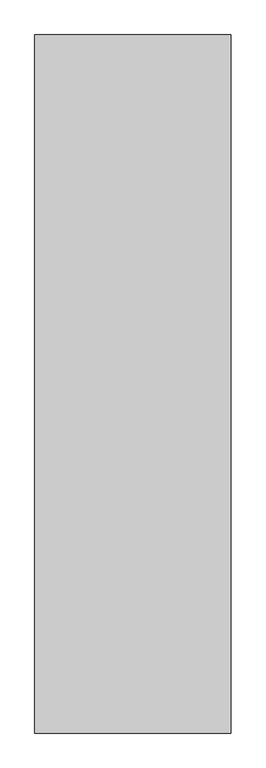
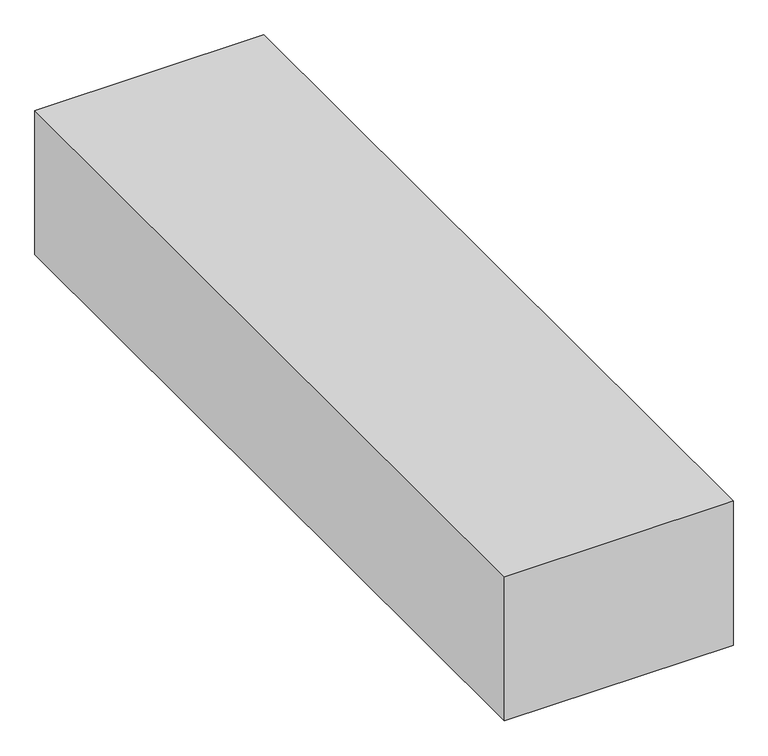
"""IFC4 building model written with IfcOpenShell, lengths in millimetres: proxy geometry, Space Planning Box_hec : Space Planning Box_hec."""

import ifcopenshell
import ifcopenshell.guid

model = None  # the IFC model being written
_history = None  # IfcOwnerHistory: only IFC2X3 demands one
_inside = {}  # id of a spatial element -> (the spatial element, [elements in it])
_under = {}  # id of a project, library or spatial element -> (it, [spatial elements below it])
_declared = {}  # id of a project -> (the project, [libraries it declares])
_typed = {}  # id of a type object -> (the type object, [elements of that type])
_made_of = {}  # id of a material, layer set ... -> (it, [elements and type objects made of it])


def new_model(schema):
    """Start an empty IFC model of exactly this schema.

    Asked for "IFC4X3", IfcOpenShell would pick the latest addendum, in which some entities
    have other attributes; the version numbers below select the first issue.
    IFC2X3 requires an IfcOwnerHistory on every rooted entity: one is made here for all.
    """
    global model, _history
    if schema == "IFC4X3":
        model = ifcopenshell.file(schema_version=(4, 3, 0, 0))
    else:
        model = ifcopenshell.file(schema=schema)
    _inside.clear()
    _under.clear()
    _declared.clear()
    _typed.clear()
    _made_of.clear()
    _history = None
    if model.schema == "IFC2X3":
        org = make("IfcOrganization", Name="unknown")
        user = make(
            "IfcPersonAndOrganization",
            ThePerson=make("IfcPerson", FamilyName="unknown"),
            TheOrganization=org,
        )
        app = make(
            "IfcApplication",
            ApplicationDeveloper=org,
            Version="unknown",
            ApplicationFullName="unknown",
            ApplicationIdentifier="unknown",
        )
        _history = make(
            "IfcOwnerHistory",
            OwningUser=user,
            OwningApplication=app,
            ChangeAction="ADDED",
            CreationDate=0,
        )
    return model


def make(cls, **values):
    """One entity of the class cls with the attributes given. An attribute that is None is left unset."""
    return model.create_entity(
        cls, **{name: value for name, value in values.items() if value is not None}
    )


def rooted(cls, **values):
    """An entity with a GlobalId (a new one), such as an element, a storey or a relation."""
    return make(cls, GlobalId=ifcopenshell.guid.new(), OwnerHistory=_history, **values)


def si_unit(unit_type, name, prefix=None):
    """IfcSIUnit, for example si_unit("LENGTHUNIT", "METRE", prefix="MILLI")."""
    return make("IfcSIUnit", UnitType=unit_type, Prefix=prefix, Name=name)


def assignment(units):
    """IfcUnitAssignment: the units of a project."""
    return None if units is None else make("IfcUnitAssignment", Units=units)


def point(xyz):
    """IfcCartesianPoint."""
    return None if xyz is None else make("IfcCartesianPoint", Coordinates=xyz)


def direction(xyz):
    """IfcDirection."""
    return None if xyz is None else make("IfcDirection", DirectionRatios=xyz)


def frame(location, z_axis=None, x_axis=None):
    """IfcAxis2Placement3D, a coordinate frame: its origin and axes. An axis left out is left unset."""
    return make(
        "IfcAxis2Placement3D",
        Location=point(location),
        Axis=direction(z_axis),
        RefDirection=direction(x_axis),
    )


def origin():
    """The frame at (0, 0, 0) with its axes left unset."""
    return frame((0.0, 0.0, 0.0))


def origin_with_axes():
    """The frame at (0, 0, 0) with the z axis (0, 0, 1) and the x axis (1, 0, 0) written out."""
    return frame((0.0, 0.0, 0.0), z_axis=(0.0, 0.0, 1.0), x_axis=(1.0, 0.0, 0.0))


def place(relative_to, where):
    """IfcLocalPlacement: puts the frame where relative to a parent placement (None: the world)."""
    return make(
        "IfcLocalPlacement", PlacementRelTo=relative_to, RelativePlacement=where
    )


def context(
    kind, dimensions, precision=None, world=None, true_north=None, identifier=None
):
    """IfcGeometricRepresentationContext, for example the 3D "Model" context."""
    return make(
        "IfcGeometricRepresentationContext",
        ContextIdentifier=identifier,
        ContextType=kind,
        CoordinateSpaceDimension=dimensions,
        Precision=precision,
        WorldCoordinateSystem=world,
        TrueNorth=true_north,
    )


def project(units=None, contexts=None):
    """IfcProject with its units and contexts."""
    return rooted(
        "IfcProject",
        Name="project",
        RepresentationContexts=contexts,
        UnitsInContext=assignment(units),
    )


def spatial(cls, under=None, at=None, **own):
    """A site, building, storey or space (cls), placed at a placement, below another one or the project."""
    s = rooted(cls, ObjectPlacement=at, **own)
    if under is not None:
        _under.setdefault(under.id(), (under, []))[1].append(s)
    return s


def polyline(points):
    """IfcPolyline through the points."""
    return make("IfcPolyline", Points=[point(p) for p in points])


def outline(outer, holes=None, kind="AREA"):
    """IfcArbitraryClosedProfileDef: a profile drawn as a closed curve; with holes, ...WithVoids."""
    if holes is None:
        return make("IfcArbitraryClosedProfileDef", ProfileType=kind, OuterCurve=outer)
    return make(
        "IfcArbitraryProfileDefWithVoids",
        ProfileType=kind,
        OuterCurve=outer,
        InnerCurves=holes,
    )


def extrude(swept, where, along, depth):
    """IfcExtrudedAreaSolid: the profile swept, set in the frame where, extruded along a direction by depth."""
    return make(
        "IfcExtrudedAreaSolid",
        SweptArea=swept,
        Position=where,
        ExtrudedDirection=direction(along),
        Depth=depth,
    )


def shape(context_of_items, identifier, shape_type, items):
    """IfcShapeRepresentation: the items that make up one representation, for example the "Body"."""
    return make(
        "IfcShapeRepresentation",
        ContextOfItems=context_of_items,
        RepresentationIdentifier=identifier,
        RepresentationType=shape_type,
        Items=items,
    )


def source(mapping_origin, context_of_items, identifier, shape_type, items):
    """IfcRepresentationMap: a shape defined once, which mapped items show again and again."""
    return make(
        "IfcRepresentationMap",
        MappingOrigin=mapping_origin,
        MappedRepresentation=shape(context_of_items, identifier, shape_type, items),
    )


def transform(
    local_origin,
    x_axis=None,
    y_axis=None,
    z_axis=None,
    scale=None,
    scale2=None,
    scale3=None,
    uniform=True,
):
    """IfcCartesianTransformationOperator3D, or its non-uniform kind. x_axis, y_axis, z_axis: its Axis1, 2, 3."""
    if uniform:
        return make(
            "IfcCartesianTransformationOperator3D",
            Axis1=direction(x_axis),
            Axis2=direction(y_axis),
            LocalOrigin=point(local_origin),
            Scale=scale,
            Axis3=direction(z_axis),
        )
    return make(
        "IfcCartesianTransformationOperator3DnonUniform",
        Axis1=direction(x_axis),
        Axis2=direction(y_axis),
        LocalOrigin=point(local_origin),
        Scale=scale,
        Axis3=direction(z_axis),
        Scale2=scale2,
        Scale3=scale3,
    )


def mapped(mapping_source, mapping_target):
    """IfcMappedItem: shows the shape of a source again, moved by a transform."""
    return make(
        "IfcMappedItem", MappingSource=mapping_source, MappingTarget=mapping_target
    )


def made_of(thing, what):
    """Note that an element or type object is made of a material, layer set ...; save() writes the relation."""
    if what is not None:
        _made_of.setdefault(what.id(), (what, []))[1].append(thing)
    return thing


def element(
    cls,
    number,
    at=None,
    inside=None,
    cuts=None,
    type_object=None,
    material=None,
    context=None,
    identifier="Body",
    shape_type=None,
    held_by="IfcProductDefinitionShape",
    body=None,
    shapes=None,
    **own,
):
    """One element of the class cls, such as IfcWall. Its Tag is "e" and its number.

    at: its placement. inside: the storey or other place that contains it. cuts: it is an
    opening in that element (IfcRelVoidsElement). A single representation is given by context,
    identifier, shape_type and body (its items); several are given by shapes. held_by: the class
    of the entity that holds the representations. save() writes the other relations.
    """
    e = rooted(cls, Tag="e%d" % number, ObjectPlacement=at, **own)
    if body is not None:
        shapes = [shape(context, identifier, shape_type, body)]
    if shapes is not None:
        e.Representation = make(held_by, Representations=shapes)
    if inside is not None:
        _inside.setdefault(inside.id(), (inside, []))[1].append(e)
    if cuts is not None:
        rooted(
            "IfcRelVoidsElement", RelatingBuildingElement=cuts, RelatedOpeningElement=e
        )
    if type_object is not None:
        _typed.setdefault(type_object.id(), (type_object, []))[1].append(e)
    return made_of(e, material)


def aggregate(whole, parts):
    """IfcRelAggregates: a whole, such as a stair, and the parts it consists of."""
    return rooted("IfcRelAggregates", RelatingObject=whole, RelatedObjects=parts)


def save(model, path):
    """Write the relations noted so far, then the file.

    IfcRelAggregates (storeys below a building ...), IfcRelContainedInSpatialStructure (elements
    in a storey), IfcRelDefinesByType, IfcRelAssociatesMaterial and IfcRelDeclares: one each for
    every whole, place, type object, material and project.
    """
    for whole, parts in _under.values():
        aggregate(whole, parts)
    for where, things in _inside.values():
        rooted(
            "IfcRelContainedInSpatialStructure",
            RelatedElements=things,
            RelatingStructure=where,
        )
    for kind, things in _typed.values():
        rooted("IfcRelDefinesByType", RelatedObjects=things, RelatingType=kind)
    for what, things in _made_of.values():
        rooted("IfcRelAssociatesMaterial", RelatedObjects=things, RelatingMaterial=what)
    for by, libraries in _declared.values():
        rooted("IfcRelDeclares", RelatingContext=by, RelatedDefinitions=libraries)
    model.write(path)


def generic_models_57c7875f(model_context):
    return source(origin(), model_context, "Body", "SweptSolid", [
        extrude(outline(polyline([(4500.0, 16000.0), (4500.0, -16000.0), (-4500.0, -16000.0), (-4500.0, 16000.0), (4500.0, 16000.0)])), origin_with_axes(), (0.0, 0.0, 1.0), 6000.0),
    ])


if __name__ == "__main__":
    model = new_model("IFC4")
    model_context = context("Model", 3, world=origin())
    ifc_project = project(units=[si_unit("LENGTHUNIT", "METRE", prefix="MILLI")], contexts=[model_context])
    site = spatial("IfcSite", under=ifc_project)
    building = spatial("IfcBuilding", under=site)
    placement = place(None, origin())
    generic_models_shape = generic_models_57c7875f(model_context)
    element("IfcBuildingElementProxy", 1, Name="Space Planning Box_hec : Space Planning Box_hec", ObjectType="Space Planning Box_hec : Space Planning Box_hec", at=placement, inside=building, context=model_context, shape_type="MappedRepresentation", body=[
        mapped(generic_models_shape, transform((0.0, 0.0, 0.0), x_axis=(1.0, 0.0, 0.0), y_axis=(0.0, 1.0, 0.0), z_axis=(0.0, 0.0, 1.0))),
    ])
    save(model, "model.ifc")

# Revit data of these elements
# Type "Space Planning Box_hec : Space Planning Box_hec"
#   Type Comments = "..."
#   Room Name [instance default] = "?"
#   Interior Finish [instance default] = ""
#   Exterior Finish [instance default] = ""
#   Department [instance default] = ""
#   Assembly Code = "..."
#   Width [instance default] = 1524 mm
#   Program Area [instance default] = 0.00 m²
#   Length [instance default] = 1524 mm
#   Height [instance default] = 1524 mm
#   Area [instance default] = 2.32258 m²
#   Fill Color [instance default] = Cyan
#   Default Elevation = 0
# Element 1 (IfcBuildingElementProxy, "Space Planning Box_hec : Space Planning Box_hec")
#   Room Name = "Central Control Room"
#   Interior Finish = "IF3"
#   Exterior Finish = "EF1"
#   Department = "CI"
#   Width = 9000 mm
#   Program Area = 288.00 m²
#   Length = 32000 mm
#   Height = 6000 mm
#   Area = 288.00 m²
#   Fill Color = Lime
#   Materials on its faces: "Lime"
# Materials
#   "Cyan": class "Generic", colour RGB 0 255 255, transparency 0.2, Cost = 0
#   "Lime": class "Generic", colour RGB 0 255 0, transparency 0.2, Cost = 0
